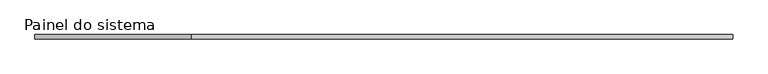
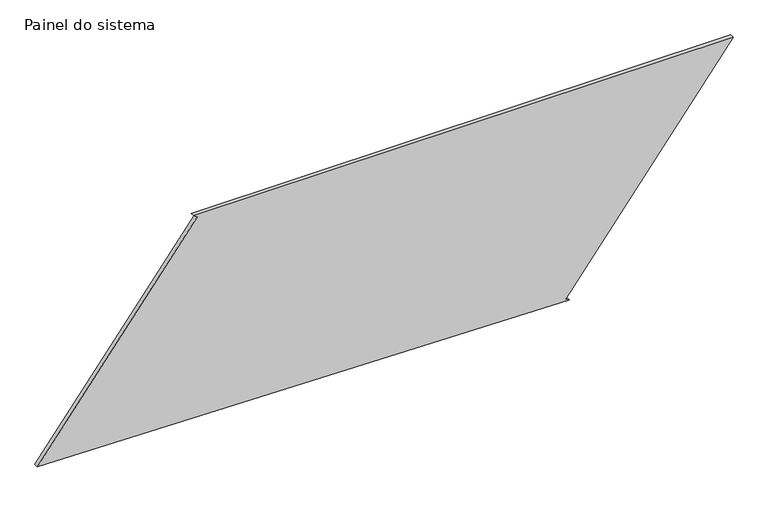
"""IFC4 building model written with IfcOpenShell, lengths in millimetres: plate geometry, Painel do sistema : Envidraçado."""

from ifc_helpers import new_model, si_unit, frame, origin, place, context, project, spatial, polyline, outline, extrude, source, transform, mapped, element, save


def painel_do_sistema_fc1bf8b4(model_context):
    return source(origin(), model_context, "Body", "SweptSolid", [
        extrude(outline(polyline([(0.0, 1094.8602664), (15.2063352, 1075.0166938), (1313.6191598, 2070.0038889), (1313.6191598, -1139.6360751), (1298.4128246, -1119.7925026), (58.4303844, -2070.0038889), (0.0, 1094.8602664)])), frame((0.0, 24.5, 0.0), z_axis=(0.0, 1.0, 0.0), x_axis=(0.0, 0.0, 1.0)), (0.0, 0.0, 1.0), 25.0),
    ])


if __name__ == "__main__":
    model = new_model("IFC4")
    model_context = context("Model", 3, world=origin())
    ifc_project = project(units=[si_unit("LENGTHUNIT", "METRE", prefix="MILLI")], contexts=[model_context])
    site = spatial("IfcSite", under=ifc_project)
    building = spatial("IfcBuilding", under=site)
    placement = place(None, origin())
    painel_do_sistema_shape = painel_do_sistema_fc1bf8b4(model_context)
    element("IfcPlate", 1, ObjectType="Painel do sistema : Envidraçado", at=placement, inside=building, context=model_context, shape_type="MappedRepresentation", body=[
        mapped(painel_do_sistema_shape, transform((0.0, 0.0, 0.0), x_axis=(1.0, 0.0, 0.0), y_axis=(0.0, 1.0, 0.0), z_axis=(0.0, 0.0, 1.0))),
    ])
    save(model, "model.ifc")

# Revit data of these elements
# Type "Painel do sistema : Envidraçado"
#   Construction Type Id = "GSP4R"
#   Analytic Construction = "Vidraça única Pilkington 1/8 pol"
#   Visual Light Transmittance = 0.9
#   Solar Heat Gain Coefficient = 0.86
#   Heat Transfer Coefficient (U) = 6.7069 W/(m²·K)
# Element 1 (IfcPlate, "Painel do sistema : Envidraçado")
#   Materials on its faces: "Vidro"
# Materials
#   "Vidro": class "Vidro", colour RGB 0 128 192, transparency 0.9, Description = "Vidro de sílica", Cost = 0
